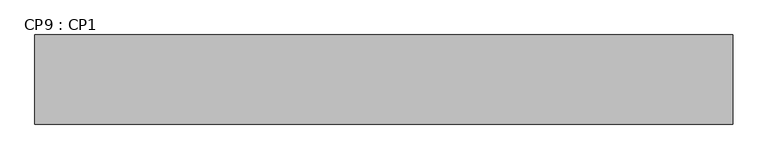
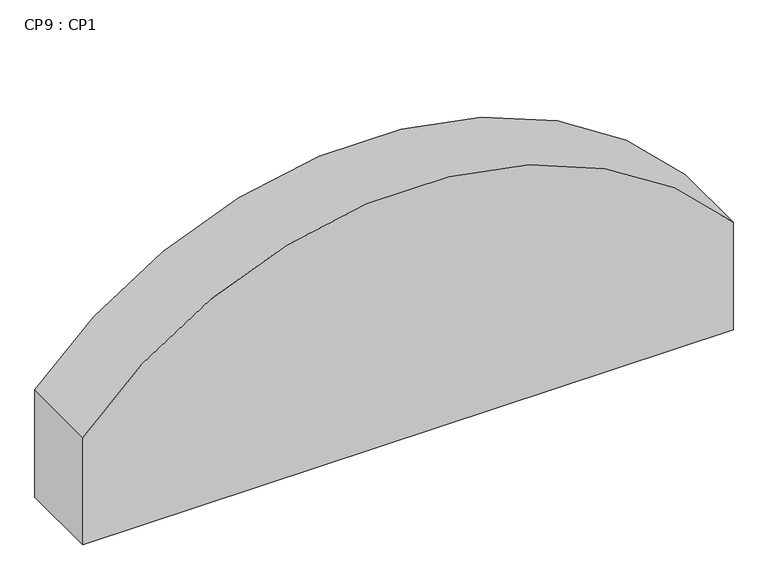
"""IFC4 building model written with IfcOpenShell, lengths in millimetres: beam geometry, CP9 : CP1."""

from ifc_helpers import new_model, si_unit, frame, origin, place, context, project, spatial, circle_curve, source, transform, mapped, element, save
from ifc_brep_helpers import plane_surface, cylinder_surface, advanced_brep


def cp9_cp1_98b19d1e(model_context):
    return source(origin(), model_context, "Body", "AdvancedBrep", [
        advanced_brep(
        [(45483.2245512, 499.6999991, 14620.0), (50183.2245511, 499.6999991, 14620.0), (50183.2245511, 499.6999991, 13800.0), (45483.2245506, 499.6999991, 13800.0), (50183.2245511, -100.2551788, 14620.0), (45483.2245512, -100.2551788, 14620.0), (45483.2245506, -100.2551788, 13800.0), (50183.2245511, -100.2551788, 13800.0)],
        [
            (0, 1, circle_curve(frame((47833.2245512, 499.6999991, 12608.2612414), z_axis=(0.0, 1.0, 0.0), x_axis=(0.0, 0.0, -1.0)), 3093.4758497)),
            (1, 2),
            (2, 3),
            (3, 0),
            (4, 5, circle_curve(frame((47833.2245512, -100.2551788, 12608.2612414), z_axis=(0.0, -1.0, 0.0), x_axis=(0.0, 0.0, -1.0)), 3093.4758497)),
            (5, 6),
            (6, 7),
            (7, 4),
            (6, 3),
            (2, 7),
            (0, 5),
            (4, 1),
        ],
        [
            plane_surface(frame((45333.2245515, 499.6999991, 13800.0), z_axis=(0.0, 1.0, 0.0), x_axis=(-1.0, 0.0, 0.0))),
            plane_surface(frame((45333.2245515, -100.2551788, 13800.0), z_axis=(0.0, -1.0, 0.0), x_axis=(1.0, 0.0, 0.0))),
            plane_surface(frame((50483.2245511, 499.6999991, 13800.0), z_axis=(0.0, 0.0, -1.0), x_axis=(0.0, -1.0, 0.0))),
            cylinder_surface(frame((47833.2245512, 20099.7448193, 12608.2612414), z_axis=(0.0, 1.0, 0.0), x_axis=(0.0, 0.0, -1.0)), 3093.4758497),
            plane_surface(frame((45483.2245506, 18587.0448193, 14620.0), z_axis=(-1.0, 0.0, 0.0), x_axis=(0.0, -1.0, 0.0))),
            plane_surface(frame((50183.2245511, 18587.0448193, 13800.0), z_axis=(1.0, 0.0, 0.0), x_axis=(0.0, -1.0, 0.0))),
        ],
        [
            (0, [[1, 2, 3, 4]]),
            (1, [[5, 6, 7, 8]]),
            (2, [[9, -3, 10, -7]]),
            (3, [[-1, 11, -5, 12]]),
            (4, [[-4, -9, -6, -11]]),
            (5, [[-2, -12, -8, -10]]),
        ],
    ),
    ])


if __name__ == "__main__":
    model = new_model("IFC4")
    model_context = context("Model", 3, world=origin())
    ifc_project = project(units=[si_unit("LENGTHUNIT", "METRE", prefix="MILLI")], contexts=[model_context])
    site = spatial("IfcSite", under=ifc_project)
    building = spatial("IfcBuilding", under=site)
    placement = place(None, origin())
    cp9_cp1_shape = cp9_cp1_98b19d1e(model_context)
    element("IfcBeam", 1, ObjectType="CP9 : CP1", at=placement, inside=building, context=model_context, shape_type="MappedRepresentation", body=[
        mapped(cp9_cp1_shape, transform((0.0, 0.0, 0.0), x_axis=(1.0, 0.0, 0.0), y_axis=(0.0, 1.0, 0.0), z_axis=(0.0, 0.0, 1.0))),
    ])
    save(model, "model.ifc")
